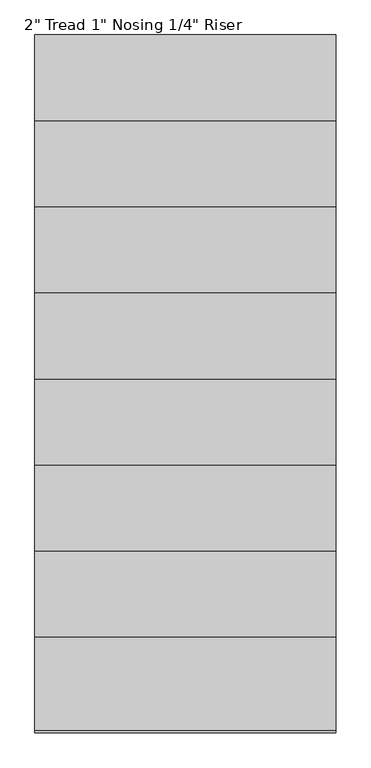
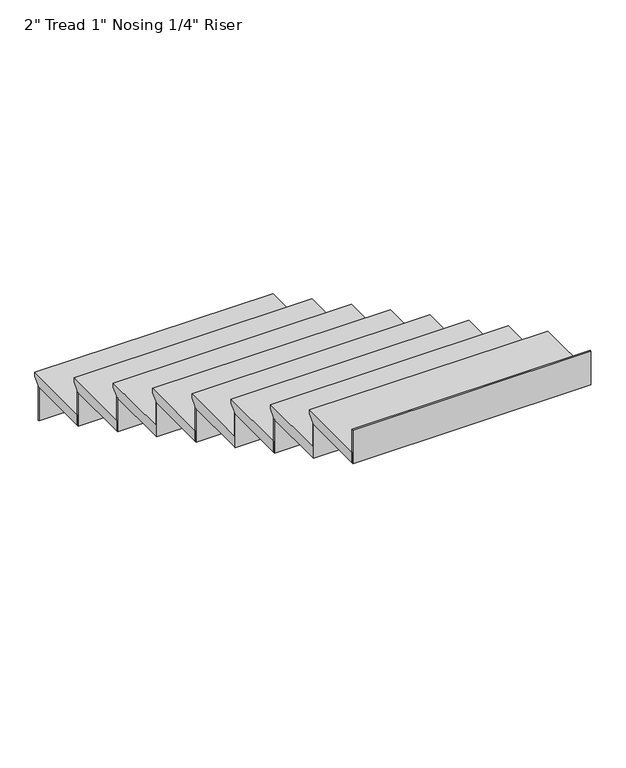
"""IFC4 building model written with IfcOpenShell, lengths in millimetres: stair flight geometry."""

import ifcopenshell
import ifcopenshell.guid

model = None  # the IFC model being written
_history = None  # IfcOwnerHistory: only IFC2X3 demands one
_inside = {}  # id of a spatial element -> (the spatial element, [elements in it])
_under = {}  # id of a project, library or spatial element -> (it, [spatial elements below it])
_declared = {}  # id of a project -> (the project, [libraries it declares])
_typed = {}  # id of a type object -> (the type object, [elements of that type])
_made_of = {}  # id of a material, layer set ... -> (it, [elements and type objects made of it])


def new_model(schema):
    """Start an empty IFC model of exactly this schema.

    Asked for "IFC4X3", IfcOpenShell would pick the latest addendum, in which some entities
    have other attributes; the version numbers below select the first issue.
    IFC2X3 requires an IfcOwnerHistory on every rooted entity: one is made here for all.
    """
    global model, _history
    if schema == "IFC4X3":
        model = ifcopenshell.file(schema_version=(4, 3, 0, 0))
    else:
        model = ifcopenshell.file(schema=schema)
    _inside.clear()
    _under.clear()
    _declared.clear()
    _typed.clear()
    _made_of.clear()
    _history = None
    if model.schema == "IFC2X3":
        org = make("IfcOrganization", Name="unknown")
        user = make(
            "IfcPersonAndOrganization",
            ThePerson=make("IfcPerson", FamilyName="unknown"),
            TheOrganization=org,
        )
        app = make(
            "IfcApplication",
            ApplicationDeveloper=org,
            Version="unknown",
            ApplicationFullName="unknown",
            ApplicationIdentifier="unknown",
        )
        _history = make(
            "IfcOwnerHistory",
            OwningUser=user,
            OwningApplication=app,
            ChangeAction="ADDED",
            CreationDate=0,
        )
    return model


def make(cls, **values):
    """One entity of the class cls with the attributes given. An attribute that is None is left unset."""
    return model.create_entity(
        cls, **{name: value for name, value in values.items() if value is not None}
    )


def rooted(cls, **values):
    """An entity with a GlobalId (a new one), such as an element, a storey or a relation."""
    return make(cls, GlobalId=ifcopenshell.guid.new(), OwnerHistory=_history, **values)


def si_unit(unit_type, name, prefix=None):
    """IfcSIUnit, for example si_unit("LENGTHUNIT", "METRE", prefix="MILLI")."""
    return make("IfcSIUnit", UnitType=unit_type, Prefix=prefix, Name=name)


def assignment(units):
    """IfcUnitAssignment: the units of a project."""
    return None if units is None else make("IfcUnitAssignment", Units=units)


def point(xyz):
    """IfcCartesianPoint."""
    return None if xyz is None else make("IfcCartesianPoint", Coordinates=xyz)


def direction(xyz):
    """IfcDirection."""
    return None if xyz is None else make("IfcDirection", DirectionRatios=xyz)


def frame(location, z_axis=None, x_axis=None):
    """IfcAxis2Placement3D, a coordinate frame: its origin and axes. An axis left out is left unset."""
    return make(
        "IfcAxis2Placement3D",
        Location=point(location),
        Axis=direction(z_axis),
        RefDirection=direction(x_axis),
    )


def origin():
    """The frame at (0, 0, 0) with its axes left unset."""
    return frame((0.0, 0.0, 0.0))


def place(relative_to, where):
    """IfcLocalPlacement: puts the frame where relative to a parent placement (None: the world)."""
    return make(
        "IfcLocalPlacement", PlacementRelTo=relative_to, RelativePlacement=where
    )


def context(
    kind, dimensions, precision=None, world=None, true_north=None, identifier=None
):
    """IfcGeometricRepresentationContext, for example the 3D "Model" context."""
    return make(
        "IfcGeometricRepresentationContext",
        ContextIdentifier=identifier,
        ContextType=kind,
        CoordinateSpaceDimension=dimensions,
        Precision=precision,
        WorldCoordinateSystem=world,
        TrueNorth=true_north,
    )


def project(units=None, contexts=None):
    """IfcProject with its units and contexts."""
    return rooted(
        "IfcProject",
        Name="project",
        RepresentationContexts=contexts,
        UnitsInContext=assignment(units),
    )


def spatial(cls, under=None, at=None, **own):
    """A site, building, storey or space (cls), placed at a placement, below another one or the project."""
    s = rooted(cls, ObjectPlacement=at, **own)
    if under is not None:
        _under.setdefault(under.id(), (under, []))[1].append(s)
    return s


def polyline(points):
    """IfcPolyline through the points."""
    return make("IfcPolyline", Points=[point(p) for p in points])


def outline(outer, holes=None, kind="AREA"):
    """IfcArbitraryClosedProfileDef: a profile drawn as a closed curve; with holes, ...WithVoids."""
    if holes is None:
        return make("IfcArbitraryClosedProfileDef", ProfileType=kind, OuterCurve=outer)
    return make(
        "IfcArbitraryProfileDefWithVoids",
        ProfileType=kind,
        OuterCurve=outer,
        InnerCurves=holes,
    )


def extrude(swept, where, along, depth):
    """IfcExtrudedAreaSolid: the profile swept, set in the frame where, extruded along a direction by depth."""
    return make(
        "IfcExtrudedAreaSolid",
        SweptArea=swept,
        Position=where,
        ExtrudedDirection=direction(along),
        Depth=depth,
    )


def shape(context_of_items, identifier, shape_type, items):
    """IfcShapeRepresentation: the items that make up one representation, for example the "Body"."""
    return make(
        "IfcShapeRepresentation",
        ContextOfItems=context_of_items,
        RepresentationIdentifier=identifier,
        RepresentationType=shape_type,
        Items=items,
    )


def source(mapping_origin, context_of_items, identifier, shape_type, items):
    """IfcRepresentationMap: a shape defined once, which mapped items show again and again."""
    return make(
        "IfcRepresentationMap",
        MappingOrigin=mapping_origin,
        MappedRepresentation=shape(context_of_items, identifier, shape_type, items),
    )


def transform(
    local_origin,
    x_axis=None,
    y_axis=None,
    z_axis=None,
    scale=None,
    scale2=None,
    scale3=None,
    uniform=True,
):
    """IfcCartesianTransformationOperator3D, or its non-uniform kind. x_axis, y_axis, z_axis: its Axis1, 2, 3."""
    if uniform:
        return make(
            "IfcCartesianTransformationOperator3D",
            Axis1=direction(x_axis),
            Axis2=direction(y_axis),
            LocalOrigin=point(local_origin),
            Scale=scale,
            Axis3=direction(z_axis),
        )
    return make(
        "IfcCartesianTransformationOperator3DnonUniform",
        Axis1=direction(x_axis),
        Axis2=direction(y_axis),
        LocalOrigin=point(local_origin),
        Scale=scale,
        Axis3=direction(z_axis),
        Scale2=scale2,
        Scale3=scale3,
    )


def mapped(mapping_source, mapping_target):
    """IfcMappedItem: shows the shape of a source again, moved by a transform."""
    return make(
        "IfcMappedItem", MappingSource=mapping_source, MappingTarget=mapping_target
    )


def made_of(thing, what):
    """Note that an element or type object is made of a material, layer set ...; save() writes the relation."""
    if what is not None:
        _made_of.setdefault(what.id(), (what, []))[1].append(thing)
    return thing


def element(
    cls,
    number,
    at=None,
    inside=None,
    cuts=None,
    type_object=None,
    material=None,
    context=None,
    identifier="Body",
    shape_type=None,
    held_by="IfcProductDefinitionShape",
    body=None,
    shapes=None,
    **own,
):
    """One element of the class cls, such as IfcWall. Its Tag is "e" and its number.

    at: its placement. inside: the storey or other place that contains it. cuts: it is an
    opening in that element (IfcRelVoidsElement). A single representation is given by context,
    identifier, shape_type and body (its items); several are given by shapes. held_by: the class
    of the entity that holds the representations. save() writes the other relations.
    """
    e = rooted(cls, Tag="e%d" % number, ObjectPlacement=at, **own)
    if body is not None:
        shapes = [shape(context, identifier, shape_type, body)]
    if shapes is not None:
        e.Representation = make(held_by, Representations=shapes)
    if inside is not None:
        _inside.setdefault(inside.id(), (inside, []))[1].append(e)
    if cuts is not None:
        rooted(
            "IfcRelVoidsElement", RelatingBuildingElement=cuts, RelatedOpeningElement=e
        )
    if type_object is not None:
        _typed.setdefault(type_object.id(), (type_object, []))[1].append(e)
    return made_of(e, material)


def aggregate(whole, parts):
    """IfcRelAggregates: a whole, such as a stair, and the parts it consists of."""
    return rooted("IfcRelAggregates", RelatingObject=whole, RelatedObjects=parts)


def save(model, path):
    """Write the relations noted so far, then the file.

    IfcRelAggregates (storeys below a building ...), IfcRelContainedInSpatialStructure (elements
    in a storey), IfcRelDefinesByType, IfcRelAssociatesMaterial and IfcRelDeclares: one each for
    every whole, place, type object, material and project.
    """
    for whole, parts in _under.values():
        aggregate(whole, parts)
    for where, things in _inside.values():
        rooted(
            "IfcRelContainedInSpatialStructure",
            RelatedElements=things,
            RelatingStructure=where,
        )
    for kind, things in _typed.values():
        rooted("IfcRelDefinesByType", RelatedObjects=things, RelatingType=kind)
    for what, things in _made_of.values():
        rooted("IfcRelAssociatesMaterial", RelatedObjects=things, RelatingMaterial=what)
    for by, libraries in _declared.values():
        rooted("IfcRelDeclares", RelatingContext=by, RelatedDefinitions=libraries)
    model.write(path)


def stair_flight_a5794d2b(model_context):
    return source(origin(), model_context, "Body", "SweptSolid", [
        extrude(outline(polyline([(-5188.3028521, 1594.5555556), (-4858.1028521, 1594.5555556), (-4858.1028521, 1575.5055556), (-4883.5028521, 1550.1055556), (-4883.5028521, 1543.7555556), (-5188.3028521, 1543.7555556), (-5188.3028521, 1594.5555556)])), frame((31596.9015552, 0.0, 0.0), z_axis=(1.0, 0.0, 0.0), x_axis=(0.0, 1.0, 0.0)), (0.0, 0.0, 1.0), 1066.8),
        extrude(outline(polyline([(31596.9015552, -4889.8528521), (31596.9015552, -4883.5028521), (32663.7015552, -4883.5028521), (32663.7015552, -4889.8528521), (31596.9015552, -4889.8528521)])), frame((0.0, 0.0, 1384.3), z_axis=(0.0, 0.0, 1.0), x_axis=(1.0, 0.0, 0.0)), (0.0, 0.0, 1.0), 159.4555556),
        extrude(outline(polyline([(31596.9015552, -5194.6528521), (31596.9015552, -5188.3028521), (32663.7015552, -5188.3028521), (32663.7015552, -5194.6528521), (31596.9015552, -5194.6528521)])), frame((0.0, 0.0, 1543.7555556), z_axis=(0.0, 0.0, 1.0), x_axis=(1.0, 0.0, 0.0)), (0.0, 0.0, 1.0), 159.4555556),
        extrude(outline(polyline([(-5493.1028521, 1754.0111111), (-5162.9028521, 1754.0111111), (-5162.9028521, 1734.9611111), (-5188.3028521, 1709.5611111), (-5188.3028521, 1703.2111111), (-5493.1028521, 1703.2111111), (-5493.1028521, 1754.0111111)])), frame((31596.9015552, 0.0, 0.0), z_axis=(1.0, 0.0, 0.0), x_axis=(0.0, 1.0, 0.0)), (0.0, 0.0, 1.0), 1066.8),
        extrude(outline(polyline([(31596.9015552, -5499.4528521), (31596.9015552, -5493.1028521), (32663.7015552, -5493.1028521), (32663.7015552, -5499.4528521), (31596.9015552, -5499.4528521)])), frame((0.0, 0.0, 1703.2111111), z_axis=(0.0, 0.0, 1.0), x_axis=(1.0, 0.0, 0.0)), (0.0, 0.0, 1.0), 159.4555556),
        extrude(outline(polyline([(-5797.9028521, 1913.4666667), (-5467.7028521, 1913.4666667), (-5467.7028521, 1894.4166667), (-5493.1028521, 1869.0166667), (-5493.1028521, 1862.6666667), (-5797.9028521, 1862.6666667), (-5797.9028521, 1913.4666667)])), frame((31596.9015552, 0.0, 0.0), z_axis=(1.0, 0.0, 0.0), x_axis=(0.0, 1.0, 0.0)), (0.0, 0.0, 1.0), 1066.8),
        extrude(outline(polyline([(31596.9015552, -5804.2528521), (31596.9015552, -5797.9028521), (32663.7015552, -5797.9028521), (32663.7015552, -5804.2528521), (31596.9015552, -5804.2528521)])), frame((0.0, 0.0, 1862.6666667), z_axis=(0.0, 0.0, 1.0), x_axis=(1.0, 0.0, 0.0)), (0.0, 0.0, 1.0), 159.4555556),
        extrude(outline(polyline([(-6102.7028521, 2072.9222222), (-5772.5028521, 2072.9222222), (-5772.5028521, 2053.8722222), (-5797.9028521, 2028.4722222), (-5797.9028521, 2022.1222222), (-6102.7028521, 2022.1222222), (-6102.7028521, 2072.9222222)])), frame((31596.9015552, 0.0, 0.0), z_axis=(1.0, 0.0, 0.0), x_axis=(0.0, 1.0, 0.0)), (0.0, 0.0, 1.0), 1066.8),
        extrude(outline(polyline([(31596.9015552, -6109.0528521), (31596.9015552, -6102.7028521), (32663.7015552, -6102.7028521), (32663.7015552, -6109.0528521), (31596.9015552, -6109.0528521)])), frame((0.0, 0.0, 2022.1222222), z_axis=(0.0, 0.0, 1.0), x_axis=(1.0, 0.0, 0.0)), (0.0, 0.0, 1.0), 159.4555556),
        extrude(outline(polyline([(-6407.5028521, 2232.3777778), (-6077.3028521, 2232.3777778), (-6077.3028521, 2213.3277778), (-6102.7028521, 2187.9277778), (-6102.7028521, 2181.5777778), (-6407.5028521, 2181.5777778), (-6407.5028521, 2232.3777778)])), frame((31596.9015552, 0.0, 0.0), z_axis=(1.0, 0.0, 0.0), x_axis=(0.0, 1.0, 0.0)), (0.0, 0.0, 1.0), 1066.8),
        extrude(outline(polyline([(31596.9015552, -6413.8528521), (31596.9015552, -6407.5028521), (32663.7015552, -6407.5028521), (32663.7015552, -6413.8528521), (31596.9015552, -6413.8528521)])), frame((0.0, 0.0, 2181.5777778), z_axis=(0.0, 0.0, 1.0), x_axis=(1.0, 0.0, 0.0)), (0.0, 0.0, 1.0), 159.4555556),
        extrude(outline(polyline([(-6712.3028521, 2391.8333333), (-6382.1028521, 2391.8333333), (-6382.1028521, 2372.7833333), (-6407.5028521, 2347.3833333), (-6407.5028521, 2341.0333333), (-6712.3028521, 2341.0333333), (-6712.3028521, 2391.8333333)])), frame((31596.9015552, 0.0, 0.0), z_axis=(1.0, 0.0, 0.0), x_axis=(0.0, 1.0, 0.0)), (0.0, 0.0, 1.0), 1066.8),
        extrude(outline(polyline([(31596.9015552, -6718.6528521), (31596.9015552, -6712.3028521), (32663.7015552, -6712.3028521), (32663.7015552, -6718.6528521), (31596.9015552, -6718.6528521)])), frame((0.0, 0.0, 2341.0333333), z_axis=(0.0, 0.0, 1.0), x_axis=(1.0, 0.0, 0.0)), (0.0, 0.0, 1.0), 159.4555556),
        extrude(outline(polyline([(-7017.1028521, 2551.2888889), (-6686.9028521, 2551.2888889), (-6686.9028521, 2532.2388889), (-6712.3028521, 2506.8388889), (-6712.3028521, 2500.4888889), (-7017.1028521, 2500.4888889), (-7017.1028521, 2551.2888889)])), frame((31596.9015552, 0.0, 0.0), z_axis=(1.0, 0.0, 0.0), x_axis=(0.0, 1.0, 0.0)), (0.0, 0.0, 1.0), 1066.8),
        extrude(outline(polyline([(31596.9015552, -7023.4528521), (31596.9015552, -7017.1028521), (32663.7015552, -7017.1028521), (32663.7015552, -7023.4528521), (31596.9015552, -7023.4528521)])), frame((0.0, 0.0, 2500.4888889), z_axis=(0.0, 0.0, 1.0), x_axis=(1.0, 0.0, 0.0)), (0.0, 0.0, 1.0), 159.4555556),
        extrude(outline(polyline([(31596.9015552, -7328.2528521), (31596.9015552, -7321.9028521), (32663.7015552, -7321.9028521), (32663.7015552, -7328.2528521), (31596.9015552, -7328.2528521)])), frame((0.0, 0.0, 2659.9444444), z_axis=(0.0, 0.0, 1.0), x_axis=(1.0, 0.0, 0.0)), (0.0, 0.0, 1.0), 159.4555556),
        extrude(outline(polyline([(-7321.9028521, 2710.7444444), (-6991.7028521, 2710.7444444), (-6991.7028521, 2691.6944444), (-7017.1028521, 2666.2944444), (-7017.1028521, 2659.9444444), (-7321.9028521, 2659.9444444), (-7321.9028521, 2710.7444444)])), frame((31596.9015552, 0.0, 0.0), z_axis=(1.0, 0.0, 0.0), x_axis=(0.0, 1.0, 0.0)), (0.0, 0.0, 1.0), 1066.8),
    ])


if __name__ == "__main__":
    model = new_model("IFC4")
    model_context = context("Model", 3, world=origin())
    ifc_project = project(units=[si_unit("LENGTHUNIT", "METRE", prefix="MILLI")], contexts=[model_context])
    site = spatial("IfcSite", under=ifc_project)
    building = spatial("IfcBuilding", under=site)
    placement = place(None, origin())
    stair_flight_shape = stair_flight_a5794d2b(model_context)
    element("IfcStairFlight", 1, ObjectType="2\" Tread 1\" Nosing 1/4\" Riser", at=placement, inside=building, context=model_context, shape_type="MappedRepresentation", body=[
        mapped(stair_flight_shape, transform((0.0, 0.0, 0.0), x_axis=(1.0, 0.0, 0.0), y_axis=(0.0, 1.0, 0.0), z_axis=(0.0, 0.0, 1.0))),
    ])
    save(model, "model.ifc")

# Revit data of these elements
# Element 1 (IfcStairFlight, "2\" Tread 1\" Nosing 1/4\" Riser")
#   Materials on its faces: "Oak Flooring", "Wood Planks"
# Materials
#   "Oak Flooring": class "Wood", colour RGB 216 169 114, transparency 0, Description = "Quercus Rubra", Cost = 0
#   "Wood Planks": class "Wood", colour RGB 129 72 39, transparency 0, Description = "Physical material.", Cost = 0
